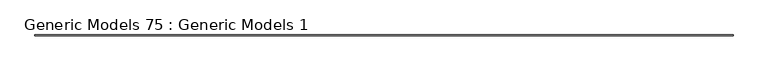
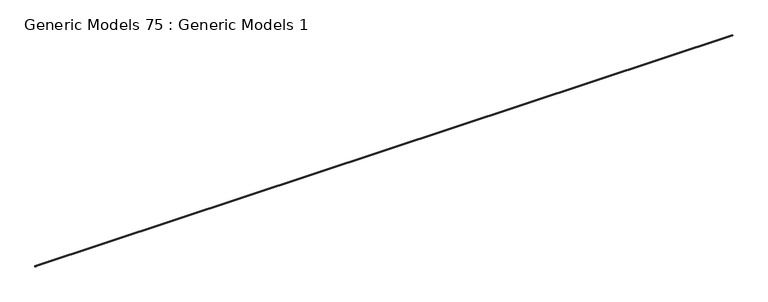
"""IFC4 building model written with IfcOpenShell, lengths in millimetres: proxy geometry, Generic Models 75 : Generic Models 1."""

from ifc_helpers import new_model, si_unit, point, frame, frame_2d, origin, place, context, project, spatial, polyline, circle_curve, trimmed, segment, composite_curve, outline, extrude, source, transform, mapped, element, save


def generic_models_75_generic_models_1_c4125e65(model_context):
    return source(origin(), model_context, "Body", "SweptSolid", [
        extrude(outline(composite_curve([segment(trimmed(circle_curve(frame_2d((-8063.4318256, 123303.525481)), 8.620055), [point((-8069.7818256, 123297.696))], [point((-8057.0818256, 123297.696))], True, "CARTESIAN"), True, "CONTINUOUS"), segment(polyline([(-8057.0818256, 123297.696), (-8057.0818256, 123288.171)]), True, "CONTINUOUS"), segment(trimmed(circle_curve(frame_2d((-8063.4318256, 123294.000481)), 8.620055), [point((-8057.0818256, 123288.171))], [point((-8069.7818256, 123288.171))], False, "CARTESIAN"), True, "CONTINUOUS"), segment(polyline([(-8069.7818256, 123288.171), (-8069.7818256, 123297.696)]), True, "CONTINUOUS")], self_intersect=False)), frame((12551.9074258, 0.0, 0.0), z_axis=(1.0, 0.0, 0.0), x_axis=(0.0, 1.0, 0.0)), (0.0, 0.0, 1.0), 12344.4),
    ])


if __name__ == "__main__":
    model = new_model("IFC4")
    model_context = context("Model", 3, world=origin())
    ifc_project = project(units=[si_unit("LENGTHUNIT", "METRE", prefix="MILLI")], contexts=[model_context])
    site = spatial("IfcSite", under=ifc_project)
    building = spatial("IfcBuilding", under=site)
    placement = place(None, origin())
    generic_models_75_generic_models_1_shape = generic_models_75_generic_models_1_c4125e65(model_context)
    element("IfcBuildingElementProxy", 1, Name="Generic Models 75 : Generic Models 1", ObjectType="Generic Models 75 : Generic Models 1", at=placement, inside=building, context=model_context, shape_type="MappedRepresentation", body=[
        mapped(generic_models_75_generic_models_1_shape, transform((0.0, 0.0, 0.0), x_axis=(1.0, 0.0, 0.0), y_axis=(0.0, 1.0, 0.0), z_axis=(0.0, 0.0, 1.0))),
    ])
    save(model, "model.ifc")

# Revit data of these elements
# Element 1 (IfcBuildingElementProxy, "Generic Models 75 : Generic Models 1")
#   Materials on its faces: "_SEALANT JOINT"
# Materials
#   "_SEALANT JOINT": class "Generic", colour RGB 190 220 196, transparency 0, Cost = 0
